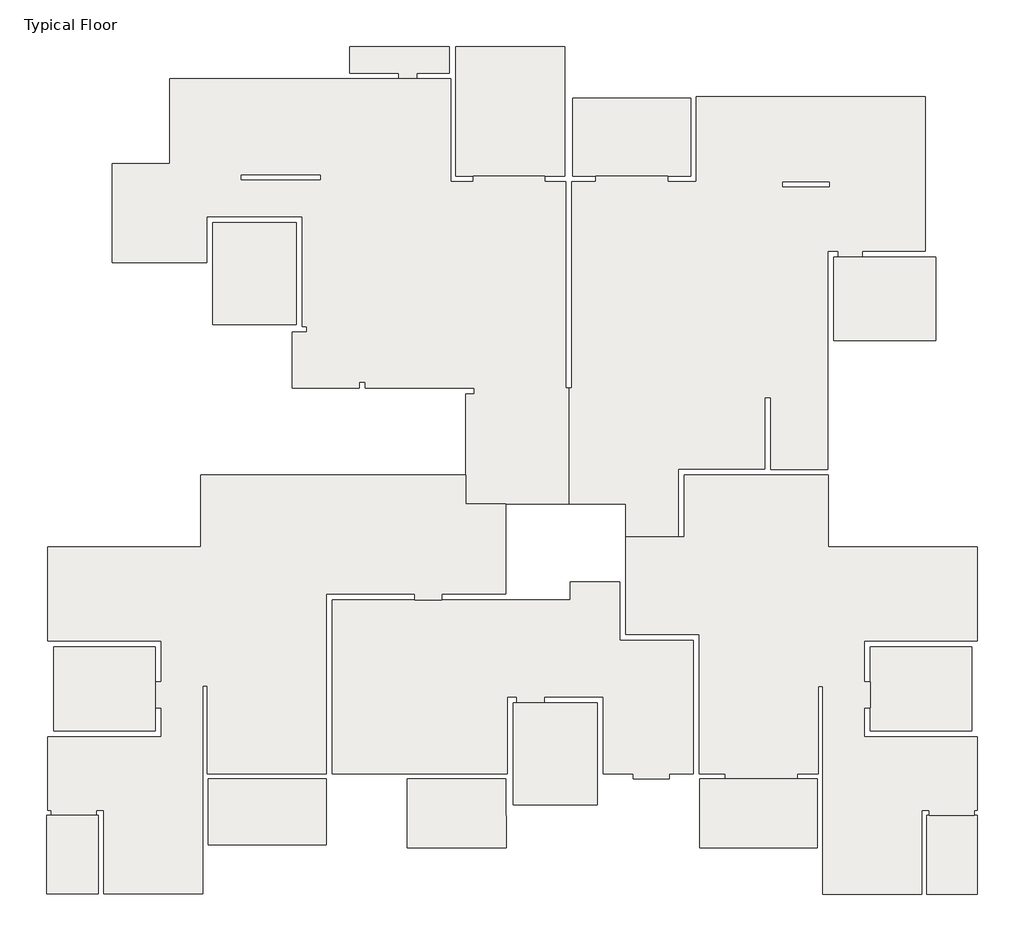
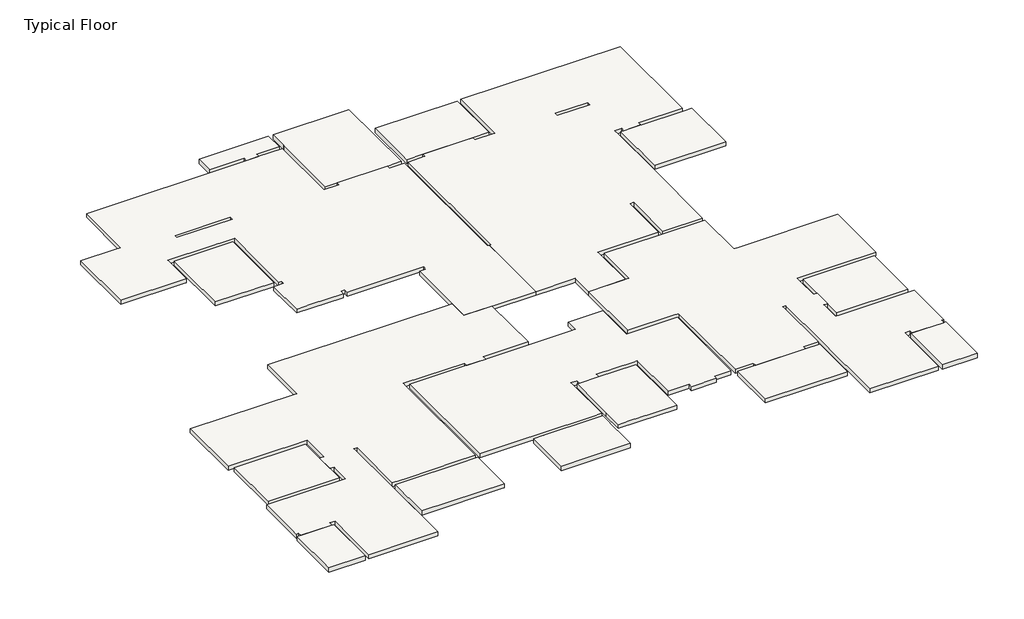
# One storey: 18 slabs.
"""IFC4 building model written with IfcOpenShell, lengths in millimetres."""

from ifc_helpers import new_model, si_unit, frame, origin, place, context, project, spatial, polyline, outline, extrude, faceted_brep, element, save

model = new_model("IFC4")

# Units and contexts
model_context = context("Model", 3, world=origin())
ifc_project = project(units=[si_unit("LENGTHUNIT", "METRE", prefix="MILLI")], contexts=[model_context])

# Site, building, storey
site = spatial("IfcSite", under=ifc_project)
building = spatial("IfcBuilding", under=site)
storey = spatial("IfcBuildingStorey", under=building, Name="Typical Floor", Elevation=3200.0)

# Slabs
placement = place(None, origin())
element("IfcSlab", 1, ObjectType="20", at=placement, inside=storey, context=model_context, shape_type="Brep", body=[
    faceted_brep([(-14926.2250005, -7113.2795537, 3000.0), (-14926.2250005, -8279.1882674, 3000.0), (-14926.2250005, -9149.744284, 3000.0), (-14926.2250005, -9913.0471886, 3000.0), (-18327.4781126, -9913.0471886, 3000.0), (-18327.4781126, -7113.2795537, 3000.0), (-14926.2250005, -7113.2795537, 3200.0), (-18327.4781126, -7113.2795537, 3200.0), (-18327.4781126, -9913.0471886, 3200.0), (-14926.2250005, -9913.0471886, 3200.0), (-14926.2250005, -9149.744284, 3200.0), (-14926.2250005, -8279.1882674, 3200.0)], [[[0, 1, 2, 3, 4, 5]], [[6, 7, 8, 9, 10, 11]], [[3, 2, 1, 0, 6, 11, 10, 9]], [[4, 3, 9, 8]], [[5, 4, 8, 7]], [[0, 5, 7, 6]]]),
])
element("IfcSlab", 2, ObjectType="20", at=placement, inside=storey, context=model_context, shape_type="Brep", body=[
    faceted_brep([(8945.0613065, -9913.0471886, 3000.0), (8945.0613065, -9149.744284, 3000.0), (8945.0613065, -8273.2795537, 3000.0), (8950.0364103, -8273.2795537, 3000.0), (8950.0364103, -7113.2795537, 3000.0), (12344.2065347, -7113.2795537, 3000.0), (12344.2065347, -9913.0471886, 3000.0), (8945.0613065, -8273.2795537, 3200.0), (8945.0613065, -9149.744284, 3200.0), (8945.0613065, -9913.0471886, 3200.0), (12344.2065347, -9913.0471886, 3200.0), (12344.2065347, -7113.2795537, 3200.0), (8950.0364103, -7113.2795537, 3200.0), (8950.0364103, -8273.2795537, 3200.0)], [[[0, 1, 2, 3, 4, 5, 6]], [[7, 8, 9, 10, 11, 12, 13]], [[9, 0, 6, 10]], [[0, 9, 8, 7, 2, 1]], [[4, 12, 11, 5]], [[3, 13, 12, 4]], [[13, 3, 2, 7]], [[6, 5, 11, 10]]]),
])
element("IfcSlab", 3, ObjectType="20", at=placement, inside=storey, context=model_context, shape_type="Brep", body=[
    faceted_brep([(-2966.5901458, -11344.051338, 3000.0), (-2966.5901458, -8982.9724998, 3000.0), (-2850.4075731, -8982.9724998, 3000.0), (-1944.0175316, -8982.9724998, 3000.0), (-164.9635897, -8982.9724998, 3000.0), (-164.9635897, -12384.2256118, 3000.0), (-2966.3411831, -12384.2256118, 3000.0), (-2966.3411831, -11344.051338, 3000.0), (-2966.5901458, -8982.9724998, 3200.0), (-2966.5901458, -11344.051338, 3200.0), (-2966.3411831, -11344.051338, 3200.0), (-2966.3411831, -11524.051338, 3200.0), (-2966.3411831, -12384.2256118, 3200.0), (-2445.6938802, -12384.2256118, 3200.0), (-1385.42832, -12384.2256118, 3200.0), (-164.9635897, -12384.2256118, 3200.0), (-164.9635897, -11524.051338, 3200.0), (-164.9635897, -11344.051338, 3200.0), (-164.9635897, -8982.9724998, 3200.0), (-1944.0175316, -8982.9724998, 3200.0), (-2850.4075731, -8982.9724998, 3200.0)], [[[0, 1, 2, 3, 4, 5, 6, 7]], [[8, 9, 10, 11, 12, 13, 14, 15, 16, 17, 18, 19, 20]], [[12, 6, 5, 15, 14, 13]], [[8, 1, 0, 9]], [[1, 8, 20, 19, 18, 4, 3, 2]], [[7, 10, 9, 0]], [[10, 7, 6, 12, 11]], [[15, 5, 4, 18, 17, 16]]]),
])
element("IfcSlab", 4, ObjectType="20", at=placement, inside=storey, context=model_context, shape_type="Brep", body=[
    faceted_brep([(11134.2812235, 3125.7328944, 3000.0), (7735.1359953, 3125.7328944, 3000.0), (7735.1359953, 5925.8407782, 3000.0), (7878.7210576, 5925.8407782, 3000.0), (7878.7210576, 5930.8407782, 3000.0), (8690.2563273, 5930.8407782, 3000.0), (8690.2563273, 5925.8407782, 3000.0), (11134.2812235, 5925.8407782, 3000.0), (7735.1359953, 3125.7328944, 3200.0), (11134.2812235, 3125.7328944, 3200.0), (11134.2812235, 5925.8407782, 3200.0), (10784.6629663, 5925.8407782, 3200.0), (8690.2563273, 5925.8407782, 3200.0), (8690.2563273, 5930.8407782, 3200.0), (7878.7210576, 5930.8407782, 3200.0), (7878.7210576, 5925.8407782, 3200.0), (7735.1359953, 5925.8407782, 3200.0)], [[[0, 1, 2, 3, 4, 5, 6, 7]], [[8, 9, 10, 11, 12, 13, 14, 15, 16]], [[13, 5, 4, 14]], [[9, 0, 7, 10]], [[1, 0, 9, 8]], [[1, 8, 16, 2]], [[10, 7, 6, 12, 11]], [[12, 6, 5, 13]], [[15, 3, 2, 16]], [[3, 15, 14, 4]]]),
])
element("IfcSlab", 5, ObjectType="20", at=placement, inside=storey, context=model_context, shape_type="Brep", body=[
    faceted_brep([(-10217.2125524, 7066.4548861, 3000.0), (-10217.2125524, 3666.4548861, 3000.0), (-13016.7312246, 3666.4548861, 3000.0), (-13016.7312246, 7066.4548861, 3000.0), (-10217.2125524, 3666.4548861, 3200.0), (-10217.2125524, 7066.4548861, 3200.0), (-13016.7312246, 7066.4548861, 3200.0), (-13016.7312246, 5736.9611102, 3200.0), (-13016.7312246, 3666.4548861, 3200.0)], [[[0, 1, 2, 3]], [[4, 5, 6, 7, 8]], [[1, 0, 5, 4]], [[1, 4, 8, 2]], [[5, 0, 3, 6]], [[2, 8, 7, 6, 3]]]),
])
element("IfcSlab", 6, ObjectType="20", at=placement, inside=storey, context=model_context, shape_type="Brep", body=[
    faceted_brep([(-9872.2125524, 3416.4548861, 3000.0), (-9872.2125524, 3596.4548861, 3000.0), (-10017.2125524, 3596.4548861, 3000.0), (-10017.2125524, 7066.4548861, 3000.0), (-10017.2125524, 7266.4548861, 3000.0), (-13016.7312246, 7266.4548861, 3000.0), (-13216.7312246, 7266.4548861, 3000.0), (-13216.7312246, 5736.9611102, 3000.0), (-13386.7312246, 5736.9611102, 3000.0), (-16367.4366188, 5736.9611102, 3000.0), (-16367.4366188, 9037.0772927, 3000.0), (-14627.1544611, 9037.0772927, 3000.0), (-14447.1544611, 9037.0772927, 3000.0), (-14447.1544611, 11886.1063384, 3000.0), (-5065.7934653, 11886.1063384, 3000.0), (-5065.7934653, 8617.6084131, 3000.0), (-5065.7934653, 8437.6084131, 3000.0), (-4315.3868263, 8437.6084131, 3000.0), (-4315.3868263, 8617.6084131, 3000.0), (-1916.615042, 8617.6084131, 3000.0), (-1916.615042, 8437.6084131, 3000.0), (-1246.7976146, 8437.6084131, 3000.0), (-1216.7976146, 8437.6084131, 3000.0), (-1216.7976146, 8435.2155047, 3000.0), (-1216.7976146, 1537.2266703, 3000.0), (-1116.7976146, 1537.2266703, 3000.0), (-1116.7976146, -2332.8480185, 3000.0), (-3216.9303947, -2332.8480185, 3000.0), (-4566.2250005, -2332.8480185, 3000.0), (-4566.2250005, -1364.051338, 3000.0), (-4566.2250005, -1089.1965662, 3000.0), (-4566.2250005, -39.4704251, 3000.0), (-4566.2250005, 1337.2266703, 3000.0), (-4266.9054985, 1337.2266703, 3000.0), (-4266.9054985, 1537.2266703, 3000.0), (-7916.2250005, 1537.2266703, 3000.0), (-7916.2250005, 1752.2266703, 3000.0), (-8116.2250005, 1752.2266703, 3000.0), (-8116.2250005, 1536.9777077, 3000.0), (-9666.1254155, 1536.9777077, 3000.0), (-10356.1254155, 1536.9777077, 3000.0), (-10356.1254155, 3416.4548861, 3000.0), (-10217.2125524, 3416.4548861, 3000.0), (-9416.4656644, 8666.4299898, 3000.0), (-12061.8598553, 8666.4299898, 3000.0), (-12061.8598553, 8516.4299898, 3000.0), (-9416.4656644, 8516.4299898, 3000.0), (-9872.2125524, 3596.4548861, 3200.0), (-9872.2125524, 3416.4548861, 3200.0), (-10217.2125524, 3416.4548861, 3200.0), (-10356.1254155, 3416.4548861, 3200.0), (-10356.1254155, 1536.9777077, 3200.0), (-9666.1254155, 1536.9777077, 3200.0), (-8116.2250005, 1536.9777077, 3200.0), (-8116.2250005, 1752.2266703, 3200.0), (-7916.2250005, 1752.2266703, 3200.0), (-7916.2250005, 1537.2266703, 3200.0), (-4266.9054985, 1537.2266703, 3200.0), (-4266.9054985, 1337.2266703, 3200.0), (-4566.2250005, 1337.2266703, 3200.0), (-4566.2250005, -39.4704251, 3200.0), (-4566.2250005, -1089.1965662, 3200.0), (-4566.2250005, -1364.051338, 3200.0), (-4566.2250005, -2332.8480185, 3200.0), (-3216.9303947, -2332.8480185, 3200.0), (-1116.7976146, -2332.8480185, 3200.0), (-1116.7976146, 1537.2266703, 3200.0), (-1216.7976146, 1537.2266703, 3200.0), (-1216.7976146, 8437.6084131, 3200.0), (-1916.615042, 8437.6084131, 3200.0), (-1916.615042, 8617.6084131, 3200.0), (-4315.3868263, 8617.6084131, 3200.0), (-4315.3868263, 8437.6084131, 3200.0), (-5065.7934653, 8437.6084131, 3200.0), (-5065.7934653, 8617.6084131, 3200.0), (-5065.7934653, 11886.1063384, 3200.0), (-6191.4034238, 11886.1063384, 3200.0), (-6790.0424279, 11886.1063384, 3200.0), (-14447.1544611, 11886.1063384, 3200.0), (-14447.1544611, 9037.0772927, 3200.0), (-14627.1544611, 9037.0772927, 3200.0), (-16367.4366188, 9037.0772927, 3200.0), (-16367.4366188, 5736.9611102, 3200.0), (-13386.7312246, 5736.9611102, 3200.0), (-13216.7312246, 5736.9611102, 3200.0), (-13216.7312246, 7266.4548861, 3200.0), (-13016.7312246, 7266.4548861, 3200.0), (-10017.2125524, 7266.4548861, 3200.0), (-10017.2125524, 7066.4548861, 3200.0), (-10017.2125524, 3596.4548861, 3200.0), (-12061.8598553, 8666.4299898, 3200.0), (-9416.4656644, 8666.4299898, 3200.0), (-9416.4656644, 8516.4299898, 3200.0), (-12061.8598553, 8516.4299898, 3200.0)], [[[0, 1, 2, 3, 4, 5, 6, 7, 8, 9, 10, 11, 12, 13, 14, 15, 16, 17, 18, 19, 20, 21, 22, 23, 24, 25, 26, 27, 28, 29, 30, 31, 32, 33, 34, 35, 36, 37, 38, 39, 40, 41, 42], [43, 44, 45, 46]], [[47, 48, 49, 50, 51, 52, 53, 54, 55, 56, 57, 58, 59, 60, 61, 62, 63, 64, 65, 66, 67, 68, 69, 70, 71, 72, 73, 74, 75, 76, 77, 78, 79, 80, 81, 82, 83, 84, 85, 86, 87, 88, 89], [90, 91, 92, 93]], [[48, 0, 42, 41, 50, 49]], [[1, 0, 48, 47]], [[2, 1, 47, 89]], [[2, 89, 88, 87, 4, 3]], [[4, 87, 86, 85, 6, 5]], [[7, 6, 85, 84]], [[7, 84, 83, 82, 9, 8]], [[10, 9, 82, 81]], [[10, 81, 80, 79, 12, 11]], [[13, 12, 79, 78]], [[14, 13, 78, 77, 76, 75]], [[14, 75, 74, 73, 16, 15]], [[17, 16, 73, 72]], [[18, 17, 72, 71]], [[19, 18, 71, 70]], [[20, 19, 70, 69]], [[22, 21, 20, 69, 68]], [[24, 23, 22, 68, 67]], [[25, 24, 67, 66]], [[26, 25, 66, 65]], [[28, 27, 26, 65, 64, 63]], [[28, 63, 62, 61, 60, 59, 32, 31, 30, 29]], [[33, 32, 59, 58]], [[34, 33, 58, 57]], [[35, 34, 57, 56]], [[36, 35, 56, 55]], [[37, 36, 55, 54]], [[38, 37, 54, 53]], [[38, 53, 52, 51, 40, 39]], [[41, 40, 51, 50]], [[44, 43, 91, 90]], [[45, 44, 90, 93]], [[46, 45, 93, 92]], [[43, 46, 92, 91]]]),
])
element("IfcSlab", 7, ObjectType="20", at=placement, inside=storey, context=model_context, shape_type="Brep", body=[
    faceted_brep([(-13417.2291499, -1364.051338, 3000.0), (-4566.2250005, -1364.051338, 3000.0), (-4566.2250005, -2332.8480185, 3000.0), (-3216.9303947, -2332.8480185, 3000.0), (-3216.9303947, -5334.7235371, 3000.0), (-5367.2208511, -5334.7235371, 3000.0), (-5367.2208511, -5534.7235371, 3000.0), (-6267.2872412, -5534.7235371, 3000.0), (-6267.2872412, -5334.7235371, 3000.0), (-9216.2167018, -5334.7235371, 3000.0), (-9216.2167018, -5534.7235371, 3000.0), (-9216.2167018, -11344.051338, 3000.0), (-10116.2830918, -11344.051338, 3000.0), (-12517.1627599, -11344.051338, 3000.0), (-13197.6689839, -11344.051338, 3000.0), (-13197.6689839, -8414.0928317, 3000.0), (-13347.6689839, -8414.0928317, 3000.0), (-13347.6689839, -11344.051338, 3000.0), (-13347.6689839, -11524.051338, 3000.0), (-13347.6689839, -15365.0637861, 3000.0), (-16646.5071582, -15365.0637861, 3000.0), (-16646.5071582, -12744.5160683, 3000.0), (-16646.5071582, -12564.5160683, 3000.0), (-16907.8847516, -12564.5160683, 3000.0), (-16907.8847516, -12744.5160683, 3000.0), (-18406.5901458, -12744.5160683, 3000.0), (-18406.5901458, -12564.5160683, 3000.0), (-18517.4781126, -12564.5160683, 3000.0), (-18517.4781126, -10113.0471886, 3000.0), (-14726.2250005, -10113.0471886, 3000.0), (-14726.2250005, -9913.0471886, 3000.0), (-14726.2250005, -9149.744284, 3000.0), (-14926.2250005, -9149.744284, 3000.0), (-14926.2250005, -8279.1882674, 3000.0), (-14726.2250005, -8279.1882674, 3000.0), (-14726.2250005, -6913.2795537, 3000.0), (-14926.2250005, -6913.2795537, 3000.0), (-18517.4781126, -6913.2795537, 3000.0), (-18517.4781126, -3764.1011305, 3000.0), (-13417.2291499, -3764.1011305, 3000.0), (-13417.2291499, -3584.1011305, 3000.0), (-4566.2250005, -1364.051338, 3200.0), (-4766.2250005, -1364.051338, 3200.0), (-9767.2291499, -1364.051338, 3200.0), (-13417.2291499, -1364.051338, 3200.0), (-13417.2291499, -3584.1011305, 3200.0), (-13417.2291499, -3764.1011305, 3200.0), (-18517.4781126, -3764.1011305, 3200.0), (-18517.4781126, -6913.2795537, 3200.0), (-14926.2250005, -6913.2795537, 3200.0), (-14726.2250005, -6913.2795537, 3200.0), (-14726.2250005, -8279.1882674, 3200.0), (-14926.2250005, -8279.1882674, 3200.0), (-14926.2250005, -9149.744284, 3200.0), (-14726.2250005, -9149.744284, 3200.0), (-14726.2250005, -9913.0471886, 3200.0), (-14726.2250005, -10113.0471886, 3200.0), (-18517.4781126, -10113.0471886, 3200.0), (-18517.4781126, -12564.5160683, 3200.0), (-18406.5901458, -12564.5160683, 3200.0), (-18406.5901458, -12744.5160683, 3200.0), (-16907.8847516, -12744.5160683, 3200.0), (-16907.8847516, -12564.5160683, 3200.0), (-16646.5071582, -12564.5160683, 3200.0), (-16646.5071582, -12744.5160683, 3200.0), (-16646.5071582, -15365.0637861, 3200.0), (-13347.6689839, -15365.0637861, 3200.0), (-13347.6689839, -11524.051338, 3200.0), (-13347.6689839, -11344.051338, 3200.0), (-13347.6689839, -8414.0928317, 3200.0), (-13197.6689839, -8414.0928317, 3200.0), (-13197.6689839, -11344.051338, 3200.0), (-12517.1627599, -11344.051338, 3200.0), (-10116.2830918, -11344.051338, 3200.0), (-9216.2167018, -11344.051338, 3200.0), (-9216.2167018, -5534.7235371, 3200.0), (-9216.2167018, -5334.7235371, 3200.0), (-6267.2872412, -5334.7235371, 3200.0), (-6267.2872412, -5534.7235371, 3200.0), (-5367.2208511, -5534.7235371, 3200.0), (-5367.2208511, -5334.7235371, 3200.0), (-3216.9303947, -5334.7235371, 3200.0), (-3216.9303947, -2332.8480185, 3200.0), (-4566.2250005, -2332.8480185, 3200.0)], [[[0, 1, 2, 3, 4, 5, 6, 7, 8, 9, 10, 11, 12, 13, 14, 15, 16, 17, 18, 19, 20, 21, 22, 23, 24, 25, 26, 27, 28, 29, 30, 31, 32, 33, 34, 35, 36, 37, 38, 39, 40]], [[41, 42, 43, 44, 45, 46, 47, 48, 49, 50, 51, 52, 53, 54, 55, 56, 57, 58, 59, 60, 61, 62, 63, 64, 65, 66, 67, 68, 69, 70, 71, 72, 73, 74, 75, 76, 77, 78, 79, 80, 81, 82, 83]], [[1, 0, 44, 43, 42, 41]], [[2, 1, 41, 83]], [[3, 2, 83, 82]], [[4, 3, 82, 81]], [[5, 4, 81, 80]], [[6, 5, 80, 79]], [[7, 6, 79, 78]], [[8, 7, 78, 77]], [[9, 8, 77, 76]], [[9, 76, 75, 74, 11, 10]], [[11, 74, 73, 72, 71, 14, 13, 12]], [[15, 14, 71, 70]], [[16, 15, 70, 69]], [[16, 69, 68, 67, 66, 19, 18, 17]], [[20, 19, 66, 65]], [[20, 65, 64, 63, 22, 21]], [[23, 22, 63, 62]], [[24, 23, 62, 61]], [[25, 24, 61, 60]], [[26, 25, 60, 59]], [[27, 26, 59, 58]], [[28, 27, 58, 57]], [[29, 28, 57, 56]], [[29, 56, 55, 54, 31, 30]], [[32, 31, 54, 53]], [[33, 32, 53, 52]], [[34, 33, 52, 51]], [[35, 34, 51, 50]], [[35, 50, 49, 48, 37, 36]], [[38, 37, 48, 47]], [[39, 38, 47, 46]], [[39, 46, 45, 44, 0, 40]]]),
])
element("IfcSlab", 8, ObjectType="20", at=placement, inside=storey, context=model_context, shape_type="Brep", body=[
    faceted_brep([(-1116.7976146, 1537.2266703, 3000.0), (-1016.7976146, 1537.2266703, 3000.0), (-1016.7976146, 8437.6084131, 3000.0), (-215.5528014, 8437.6084131, 3000.0), (-215.5528014, 8617.6084131, 3000.0), (2183.2189829, 8617.6084131, 3000.0), (2183.2189829, 8437.6084131, 3000.0), (3133.8745845, 8437.6084131, 3000.0), (3133.8745845, 8617.6084131, 3000.0), (3133.8745845, 11276.9279151, 3000.0), (10784.6629663, 11276.9279151, 3000.0), (10784.6629663, 6125.8407782, 3000.0), (8690.2563273, 6125.8407782, 3000.0), (8690.2563273, 5930.8407782, 3000.0), (7878.7210576, 5930.8407782, 3000.0), (7878.7210576, 6125.8407782, 3000.0), (7535.1359953, 6125.8407782, 3000.0), (7535.1359953, 5925.8407782, 3000.0), (7535.1359953, 2875.7328944, 3000.0), (7535.1359953, -1184.051338, 3000.0), (5633.824792, -1184.051338, 3000.0), (5633.824792, 1223.1519815, 3000.0), (5433.824792, 1223.1519815, 3000.0), (5433.824792, -1164.051338, 3000.0), (2535.2355804, -1164.051338, 3000.0), (2535.2355804, -1364.051338, 3000.0), (2535.2355804, -3433.1633712, 3000.0), (783.3351654, -3433.1633712, 3000.0), (783.3351654, -2332.8480185, 3000.0), (583.3351654, -2332.8480185, 3000.0), (-1116.7976146, -2332.8480185, 3000.0), (7585.7252069, 8425.7909857, 3000.0), (6036.4306011, 8425.7909857, 3000.0), (6036.4306011, 8275.7909857, 3000.0), (7585.7252069, 8275.7909857, 3000.0), (-1016.7976146, 1537.2266703, 3200.0), (-1116.7976146, 1537.2266703, 3200.0), (-1116.7976146, -2332.8480185, 3200.0), (583.3351654, -2332.8480185, 3200.0), (783.3351654, -2332.8480185, 3200.0), (783.3351654, -3433.1633712, 3200.0), (2535.2355804, -3433.1633712, 3200.0), (2535.2355804, -1364.051338, 3200.0), (2535.2355804, -1164.051338, 3200.0), (5433.824792, -1164.051338, 3200.0), (5433.824792, 1223.1519815, 3200.0), (5633.824792, 1223.1519815, 3200.0), (5633.824792, -1184.051338, 3200.0), (7535.1359953, -1184.051338, 3200.0), (7535.1359953, 2875.7328944, 3200.0), (7535.1359953, 5925.8407782, 3200.0), (7535.1359953, 6125.8407782, 3200.0), (7878.7210576, 6125.8407782, 3200.0), (7878.7210576, 5930.8407782, 3200.0), (8690.2563273, 5930.8407782, 3200.0), (8690.2563273, 6125.8407782, 3200.0), (10784.6629663, 6125.8407782, 3200.0), (10784.6629663, 6175.8407782, 3200.0), (10784.6629663, 11276.9279151, 3200.0), (3133.8745845, 11276.9279151, 3200.0), (3133.8745845, 8617.6084131, 3200.0), (3133.8745845, 8437.6084131, 3200.0), (2183.2189829, 8437.6084131, 3200.0), (2183.2189829, 8617.6084131, 3200.0), (-215.5528014, 8617.6084131, 3200.0), (-215.5528014, 8437.6084131, 3200.0), (-1016.7976146, 8437.6084131, 3200.0), (6036.4306011, 8425.7909857, 3200.0), (7585.7252069, 8425.7909857, 3200.0), (7585.7252069, 8275.7909857, 3200.0), (6036.4306011, 8275.7909857, 3200.0)], [[[0, 1, 2, 3, 4, 5, 6, 7, 8, 9, 10, 11, 12, 13, 14, 15, 16, 17, 18, 19, 20, 21, 22, 23, 24, 25, 26, 27, 28, 29, 30], [31, 32, 33, 34]], [[35, 36, 37, 38, 39, 40, 41, 42, 43, 44, 45, 46, 47, 48, 49, 50, 51, 52, 53, 54, 55, 56, 57, 58, 59, 60, 61, 62, 63, 64, 65, 66], [67, 68, 69, 70]], [[1, 0, 36, 35]], [[2, 1, 35, 66]], [[3, 2, 66, 65]], [[4, 3, 65, 64]], [[5, 4, 64, 63]], [[6, 5, 63, 62]], [[7, 6, 62, 61]], [[7, 61, 60, 59, 9, 8]], [[10, 9, 59, 58]], [[11, 10, 58, 57, 56]], [[12, 11, 56, 55]], [[12, 55, 54, 13]], [[52, 15, 14, 53]], [[16, 15, 52, 51]], [[16, 51, 50, 49, 18, 17]], [[20, 19, 48, 47]], [[21, 20, 47, 46]], [[22, 21, 46, 45]], [[23, 22, 45, 44]], [[24, 23, 44, 43]], [[24, 43, 42, 41, 26, 25]], [[27, 26, 41, 40]], [[28, 27, 40, 39]], [[28, 39, 38, 37, 30, 29]], [[0, 30, 37, 36]], [[19, 18, 49, 48]], [[32, 31, 68, 67]], [[33, 32, 67, 70]], [[34, 33, 70, 69]], [[31, 34, 69, 68]], [[14, 13, 54, 53]]]),
])
element("IfcSlab", 9, ObjectType="20", at=placement, inside=storey, context=model_context, shape_type="Brep", body=[
    faceted_brep([(2735.2355804, -3433.1633712, 3000.0), (2735.2355804, -1364.051338, 3000.0), (7555.384958, -1364.051338, 3000.0), (7555.384958, -3764.1011305, 3000.0), (7735.384958, -3764.1011305, 3000.0), (12534.2065347, -3764.1011305, 3000.0), (12534.2065347, -6913.2795537, 3000.0), (8750.0364103, -6913.2795537, 3000.0), (8750.0364103, -7113.2795537, 3000.0), (8750.0364103, -8273.2795537, 3000.0), (8945.0613065, -8273.2795537, 3000.0), (8945.0613065, -9149.744284, 3000.0), (8745.0613065, -9149.744284, 3000.0), (8745.0613065, -10113.0471886, 3000.0), (8945.0613065, -10113.0471886, 3000.0), (12534.2065347, -10113.0471886, 3000.0), (12534.2065347, -12564.5160683, 3000.0), (12429.6422194, -12564.5160683, 3000.0), (12429.6422194, -12744.5160683, 3000.0), (10930.9368252, -12744.5160683, 3000.0), (10930.9368252, -12564.5160683, 3000.0), (10665.3434642, -12564.5160683, 3000.0), (10665.3434642, -12744.5160683, 3000.0), (10665.3434642, -15369.5160683, 3000.0), (7365.3434642, -15369.5160683, 3000.0), (7365.3434642, -11434.051338, 3000.0), (7365.3434642, -8419.051338, 3000.0), (7215.3434642, -8419.051338, 3000.0), (7215.3434642, -11344.051338, 3000.0), (6514.9202277, -11344.051338, 3000.0), (6514.9202277, -11524.051338, 3000.0), (4114.0405596, -11524.051338, 3000.0), (4114.0405596, -11344.051338, 3000.0), (3235.0530078, -11344.051338, 3000.0), (3235.0530078, -6683.5202176, 3000.0), (3035.0530078, -6683.5202176, 3000.0), (783.3351654, -6683.5202176, 3000.0), (783.3351654, -3433.1633712, 3000.0), (2535.2355804, -3433.1633712, 3000.0), (2735.2355804, -1364.051338, 3200.0), (2735.2355804, -3433.1633712, 3200.0), (2535.2355804, -3433.1633712, 3200.0), (783.3351654, -3433.1633712, 3200.0), (783.3351654, -6683.5202176, 3200.0), (3035.0530078, -6683.5202176, 3200.0), (3235.0530078, -6683.5202176, 3200.0), (3235.0530078, -11344.051338, 3200.0), (4114.0405596, -11344.051338, 3200.0), (4114.0405596, -11524.051338, 3200.0), (6514.9202277, -11524.051338, 3200.0), (6514.9202277, -11344.051338, 3200.0), (7215.3434642, -11344.051338, 3200.0), (7215.3434642, -8419.051338, 3200.0), (7365.3434642, -8419.051338, 3200.0), (7365.3434642, -11434.051338, 3200.0), (7365.3434642, -15369.5160683, 3200.0), (10665.3434642, -15369.5160683, 3200.0), (10665.3434642, -12744.5160683, 3200.0), (10665.3434642, -12564.5160683, 3200.0), (10930.9368252, -12564.5160683, 3200.0), (10930.9368252, -12744.5160683, 3200.0), (12429.6422194, -12744.5160683, 3200.0), (12429.6422194, -12564.5160683, 3200.0), (12534.2065347, -12564.5160683, 3200.0), (12534.2065347, -10113.0471886, 3200.0), (8945.0613065, -10113.0471886, 3200.0), (8745.0613065, -10113.0471886, 3200.0), (8745.0613065, -9149.744284, 3200.0), (8945.0613065, -9149.744284, 3200.0), (8945.0613065, -8273.2795537, 3200.0), (8750.0364103, -8273.2795537, 3200.0), (8750.0364103, -7113.2795537, 3200.0), (8750.0364103, -6913.2795537, 3200.0), (12534.2065347, -6913.2795537, 3200.0), (12534.2065347, -3764.1011305, 3200.0), (7735.384958, -3764.1011305, 3200.0), (7555.384958, -3764.1011305, 3200.0), (7555.384958, -1364.051338, 3200.0), (5433.824792, -1364.051338, 3200.0)], [[[0, 1, 2, 3, 4, 5, 6, 7, 8, 9, 10, 11, 12, 13, 14, 15, 16, 17, 18, 19, 20, 21, 22, 23, 24, 25, 26, 27, 28, 29, 30, 31, 32, 33, 34, 35, 36, 37, 38]], [[39, 40, 41, 42, 43, 44, 45, 46, 47, 48, 49, 50, 51, 52, 53, 54, 55, 56, 57, 58, 59, 60, 61, 62, 63, 64, 65, 66, 67, 68, 69, 70, 71, 72, 73, 74, 75, 76, 77, 78]], [[1, 0, 40, 39]], [[2, 1, 39, 78, 77]], [[3, 2, 77, 76]], [[3, 76, 75, 74, 5, 4]], [[6, 5, 74, 73]], [[7, 6, 73, 72]], [[7, 72, 71, 70, 9, 8]], [[9, 70, 69, 10]], [[67, 12, 11, 68]], [[13, 12, 67, 66]], [[13, 66, 65, 64, 15, 14]], [[16, 15, 64, 63]], [[17, 16, 63, 62]], [[18, 17, 62, 61]], [[19, 18, 61, 60]], [[20, 19, 60, 59]], [[21, 20, 59, 58]], [[21, 58, 57, 56, 23, 22]], [[24, 23, 56, 55]], [[24, 55, 54, 53, 26, 25]], [[27, 26, 53, 52]], [[28, 27, 52, 51]], [[29, 28, 51, 50]], [[30, 29, 50, 49]], [[31, 30, 49, 48]], [[32, 31, 48, 47]], [[33, 32, 47, 46]], [[34, 33, 46, 45]], [[34, 45, 44, 43, 36, 35]], [[37, 36, 43, 42]], [[37, 42, 41, 40, 0, 38]], [[11, 10, 69, 68]]]),
])
element("IfcSlab", 10, ObjectType="20", at=placement, inside=storey, context=model_context, shape_type="Brep", body=[
    faceted_brep([(-9016.2167018, -11344.051338, 3000.0), (-9016.2167018, -5534.7235371, 3000.0), (-6267.2872412, -5534.7235371, 3000.0), (-5367.2208511, -5534.7235371, 3000.0), (-1265.2789424, -5534.7235371, 3000.0), (-1065.2789424, -5534.7235371, 3000.0), (-1065.2789424, -4933.7276865, 3000.0), (583.3351654, -4933.7276865, 3000.0), (583.3351654, -6683.5202176, 3000.0), (583.3351654, -6883.5202176, 3000.0), (3035.0530078, -6883.5202176, 3000.0), (3035.0530078, -11344.051338, 3000.0), (2233.8081945, -11344.051338, 3000.0), (2233.8081945, -11524.051338, 3000.0), (1034.4223024, -11524.051338, 3000.0), (1034.4223024, -11344.051338, 3000.0), (35.0364103, -11344.051338, 3000.0), (35.0364103, -8782.9724998, 3000.0), (-164.9635897, -8782.9724998, 3000.0), (-1944.0175316, -8782.9724998, 3000.0), (-1944.0175316, -8982.9724998, 3000.0), (-2850.4075731, -8982.9724998, 3000.0), (-2850.4075731, -8782.9724998, 3000.0), (-3166.5901458, -8782.9724998, 3000.0), (-3166.5901458, -8982.9724998, 3000.0), (-3166.5901458, -11344.051338, 3000.0), (-3636.648237, -11344.051338, 3000.0), (-6035.4200213, -11344.051338, 3000.0), (-7066.175208, -11344.051338, 3000.0), (-8566.988486, -11344.051338, 3000.0), (-9016.2167018, -5534.7235371, 3200.0), (-9016.2167018, -11344.051338, 3200.0), (-8566.988486, -11344.051338, 3200.0), (-7066.175208, -11344.051338, 3200.0), (-6035.4200213, -11344.051338, 3200.0), (-3636.648237, -11344.051338, 3200.0), (-3166.5901458, -11344.051338, 3200.0), (-3166.5901458, -8982.9724998, 3200.0), (-3166.5901458, -8782.9724998, 3200.0), (-2850.4075731, -8782.9724998, 3200.0), (-2850.4075731, -8982.9724998, 3200.0), (-1944.0175316, -8982.9724998, 3200.0), (-1944.0175316, -8782.9724998, 3200.0), (-164.9635897, -8782.9724998, 3200.0), (35.0364103, -8782.9724998, 3200.0), (35.0364103, -11344.051338, 3200.0), (1034.4223024, -11344.051338, 3200.0), (1034.4223024, -11524.051338, 3200.0), (2233.8081945, -11524.051338, 3200.0), (2233.8081945, -11344.051338, 3200.0), (3035.0530078, -11344.051338, 3200.0), (3035.0530078, -6883.5202176, 3200.0), (583.3351654, -6883.5202176, 3200.0), (583.3351654, -6683.5202176, 3200.0), (583.3351654, -4933.7276865, 3200.0), (-1065.2789424, -4933.7276865, 3200.0), (-1065.2789424, -5534.7235371, 3200.0), (-1265.2789424, -5534.7235371, 3200.0), (-5367.2208511, -5534.7235371, 3200.0), (-6267.2872412, -5534.7235371, 3200.0)], [[[0, 1, 2, 3, 4, 5, 6, 7, 8, 9, 10, 11, 12, 13, 14, 15, 16, 17, 18, 19, 20, 21, 22, 23, 24, 25, 26, 27, 28, 29]], [[30, 31, 32, 33, 34, 35, 36, 37, 38, 39, 40, 41, 42, 43, 44, 45, 46, 47, 48, 49, 50, 51, 52, 53, 54, 55, 56, 57, 58, 59]], [[1, 0, 31, 30]], [[1, 30, 59, 58, 3, 2]], [[3, 58, 57, 56, 5, 4]], [[6, 5, 56, 55]], [[7, 6, 55, 54]], [[7, 54, 53, 52, 9, 8]], [[10, 9, 52, 51]], [[11, 10, 51, 50]], [[12, 11, 50, 49]], [[13, 12, 49, 48]], [[14, 13, 48, 47]], [[15, 14, 47, 46]], [[16, 15, 46, 45]], [[17, 16, 45, 44]], [[17, 44, 43, 42, 19, 18]], [[20, 19, 42, 41]], [[21, 20, 41, 40]], [[22, 21, 40, 39]], [[23, 22, 39, 38]], [[23, 38, 37, 36, 25, 24]], [[25, 36, 35, 34, 33, 32, 31, 0, 29, 28, 27, 26]]]),
])
element("IfcSlab", 11, ObjectType="22", at=placement, inside=storey, context=model_context, shape_type="Brep", body=[
    faceted_brep([(-16826.5071582, -15365.0637861, 2980.0), (-18561.2442958, -15365.0637861, 2980.0), (-18561.2442958, -12744.5160683, 2980.0), (-16826.5071582, -12744.5160683, 2980.0), (-16826.5071582, -15365.0637861, 3200.0), (-16826.5071582, -12744.5160683, 3200.0), (-16907.8847516, -12744.5160683, 3200.0), (-18406.5901458, -12744.5160683, 3200.0), (-18561.2442958, -12744.5160683, 3200.0), (-18561.2442958, -15365.0637861, 3200.0)], [[[0, 1, 2, 3]], [[4, 5, 6, 7, 8, 9]], [[1, 0, 4, 9]], [[2, 1, 9, 8]], [[3, 2, 8, 7, 6, 5]], [[0, 3, 5, 4]]]),
])
element("IfcSlab", 12, ObjectType="22", at=placement, inside=storey, context=model_context, shape_type="Brep", body=[
    faceted_brep([(12534.2065347, -12744.5160683, 2980.0), (12534.2065347, -15369.5160683, 2980.0), (10845.3434642, -15369.5160683, 2980.0), (10845.3434642, -12744.5160683, 2980.0), (12534.2065347, -12744.5160683, 3200.0), (12429.6422194, -12744.5160683, 3200.0), (10930.9368252, -12744.5160683, 3200.0), (10845.3434642, -12744.5160683, 3200.0), (10845.3434642, -15369.5160683, 3200.0), (12534.2065347, -15369.5160683, 3200.0)], [[[0, 1, 2, 3]], [[4, 5, 6, 7, 8, 9]], [[1, 0, 4, 9]], [[2, 1, 9, 8]], [[3, 2, 8, 7]], [[0, 3, 7, 6, 5, 4]]]),
])
element("IfcSlab", 13, ObjectType="22", at=placement, inside=storey, context=model_context, shape_type="Brep", body=[
    faceted_brep([(-3211.3411831, -13814.491172, 2980.0), (-3220.4458666, -13814.491172, 2980.0), (-6516.0175316, -13814.491172, 2980.0), (-6516.0175316, -11524.051338, 2980.0), (-6035.4200213, -11524.051338, 2980.0), (-6035.4200213, -11519.051338, 2980.0), (-3636.648237, -11519.051338, 2980.0), (-3636.648237, -11524.051338, 2980.0), (-3216.3411831, -11524.051338, 2980.0), (-3216.3411831, -12636.8603469, 2980.0), (-3216.3411831, -12754.2256118, 2980.0), (-3211.3411831, -12754.2256118, 2980.0), (-6516.0175316, -13814.491172, 3200.0), (-3220.4458666, -13814.491172, 3200.0), (-3211.3411831, -13814.491172, 3200.0), (-3211.3411831, -12754.2256118, 3200.0), (-3216.3411831, -12754.2256118, 3200.0), (-3216.3411831, -11524.051338, 3200.0), (-3636.648237, -11524.051338, 3200.0), (-3636.648237, -11519.051338, 3200.0), (-6035.4200213, -11519.051338, 3200.0), (-6035.4200213, -11524.051338, 3200.0), (-6516.0175316, -11524.051338, 3200.0), (-6516.0175316, -13068.3003006, 3200.0)], [[[0, 1, 2, 3, 4, 5, 6, 7, 8, 9, 10, 11]], [[12, 13, 14, 15, 16, 17, 18, 19, 20, 21, 22, 23]], [[14, 0, 11, 15]], [[2, 1, 0, 14, 13, 12]], [[2, 12, 23, 22, 3]], [[19, 6, 5, 20]], [[7, 18, 17, 8]], [[18, 7, 6, 19]], [[21, 4, 3, 22]], [[4, 21, 20, 5]], [[16, 10, 9, 8, 17]], [[10, 16, 15, 11]]]),
])
element("IfcSlab", 14, ObjectType="22", at=placement, inside=storey, context=model_context, shape_type="Brep", body=[
    faceted_brep([(7185.3434642, -11524.051338, 2980.0), (7185.3434642, -13814.491172, 2980.0), (3265.0530078, -13814.491172, 2980.0), (3265.0530078, -11524.051338, 2980.0), (7185.3434642, -13814.491172, 3200.0), (7185.3434642, -11524.051338, 3200.0), (6514.9202277, -11524.051338, 3200.0), (4114.0405596, -11524.051338, 3200.0), (3265.0530078, -11524.051338, 3200.0), (3265.0530078, -13814.491172, 3200.0)], [[[0, 1, 2, 3]], [[4, 5, 6, 7, 8, 9]], [[1, 0, 5, 4]], [[2, 1, 4, 9]], [[3, 2, 9, 8]], [[0, 3, 8, 7, 6, 5]]]),
])
element("IfcSlab", 15, ObjectType="22", at=placement, inside=storey, context=model_context, shape_type="Brep", body=[
    faceted_brep([(-9211.2167018, -13713.3127488, 2980.0), (-9216.2167018, -13713.3127488, 2980.0), (-13167.6689839, -13713.3127488, 2980.0), (-13167.6689839, -11524.051338, 2980.0), (-9216.2167018, -11524.051338, 2980.0), (-9216.2167018, -13068.3003006, 2980.0), (-9211.2167018, -13068.3003006, 2980.0), (-13167.6689839, -13713.3127488, 3200.0), (-9211.2167018, -13713.3127488, 3200.0), (-9211.2167018, -13068.3003006, 3200.0), (-9216.2167018, -13068.3003006, 3200.0), (-9216.2167018, -11524.051338, 3200.0), (-10116.2830918, -11524.051338, 3200.0), (-12517.1627599, -11524.051338, 3200.0), (-13167.6689839, -11524.051338, 3200.0)], [[[0, 1, 2, 3, 4, 5, 6]], [[7, 8, 9, 10, 11, 12, 13, 14]], [[8, 0, 6, 9]], [[2, 1, 0, 8, 7]], [[3, 2, 7, 14]], [[3, 14, 13, 12, 11, 4]], [[10, 5, 4, 11]], [[5, 10, 9, 6]]]),
])
element("IfcSlab", 16, ObjectType="22", at=placement, inside=storey, context=model_context, shape_type="SweptSolid", body=[
    extrude(outline(polyline([(-8435.5693989, 12957.7411932), (-5116.3826769, 12957.7411932), (-5116.3826769, 12066.1063384), (-6191.4034238, 12066.1063384), (-6191.4034238, 11886.1063384), (-6790.0424279, 11886.1063384), (-6790.0424279, 12066.1063384), (-8435.5693989, 12066.1063384), (-8435.5693989, 12957.7411932)])), frame((0.0, 0.0, 2980.0), z_axis=(0.0, 0.0, 1.0), x_axis=(1.0, 0.0, 0.0)), (0.0, 0.0, 1.0), 220.0),
])
element("IfcSlab", 17, ObjectType="22", at=placement, inside=storey, context=model_context, shape_type="Brep", body=[
    faceted_brep([(-1246.7976146, 12957.7411932, 2980.0), (-1246.7976146, 8617.6084131, 2980.0), (-4885.7934653, 8617.6084131, 2980.0), (-4885.7934653, 12066.1063384, 2980.0), (-4886.3826769, 12066.1063384, 2980.0), (-4886.3826769, 12957.7411932, 2980.0), (-1246.7976146, 8617.6084131, 3200.0), (-1246.7976146, 12957.7411932, 3200.0), (-4886.3826769, 12957.7411932, 3200.0), (-4886.3826769, 12066.1063384, 3200.0), (-4885.7934653, 12066.1063384, 3200.0), (-4885.7934653, 8617.6084131, 3200.0), (-4315.3868263, 8617.6084131, 3200.0), (-1916.615042, 8617.6084131, 3200.0)], [[[0, 1, 2, 3, 4, 5]], [[6, 7, 8, 9, 10, 11, 12, 13]], [[1, 0, 7, 6]], [[1, 6, 13, 12, 11, 2]], [[8, 5, 4, 9]], [[0, 5, 8, 7]], [[10, 3, 2, 11]], [[3, 10, 9, 4]]]),
])
element("IfcSlab", 18, ObjectType="22", at=placement, inside=storey, context=model_context, shape_type="Brep", body=[
    faceted_brep([(2953.8745845, 11237.7079981, 2980.0), (2953.8745845, 8617.6084131, 2980.0), (-986.7976146, 8617.6084131, 2980.0), (-986.7976146, 11237.7079981, 2980.0), (2953.8745845, 8617.6084131, 3200.0), (2953.8745845, 11237.7079981, 3200.0), (-986.7976146, 11237.7079981, 3200.0), (-986.7976146, 8617.6084131, 3200.0), (-215.5528014, 8617.6084131, 3200.0), (2183.2189829, 8617.6084131, 3200.0)], [[[0, 1, 2, 3]], [[4, 5, 6, 7, 8, 9]], [[1, 0, 5, 4]], [[2, 1, 4, 9, 8, 7]], [[3, 2, 7, 6]], [[0, 3, 6, 5]]]),
])

save(model, "model.ifc")

# Revit data of these elements
# Type "20"
#   Function = 0
#   Layers, outside or top first: 20 cm "Concrete" (function 1)
# Type "22"
#   Function = 0
#   Layers, outside or top first: 22 cm "Concrete" (function 1)
# Element 1 (IfcSlab, "20")
#   Mark = "S9"
#   SOFiSTiK_AMG_Comments = ""
#   Height Offset From Level = 0 cm
#   built-in parameter 1001954 = 1
#   SOFiSTiK_AMG_Scheduled = yes
#   SOFiSTiK_AMG_Adjusted = yes
#   Phase Created = New Construction
#   Materials on its faces: "Concrete"
# Element 2 (IfcSlab, "20")
#   Mark = "S10"
#   SOFiSTiK_AMG_Comments = ""
#   Height Offset From Level = 0 cm
#   built-in parameter 1001954 = 1
#   SOFiSTiK_AMG_Scheduled = yes
#   SOFiSTiK_AMG_Adjusted = yes
#   Phase Created = New Construction
#   Materials on its faces: "Concrete"
# Element 3 (IfcSlab, "20")
#   Mark = "S11"
#   SOFiSTiK_AMG_Comments = ""
#   Height Offset From Level = 0 cm
#   built-in parameter 1001954 = 1
#   SOFiSTiK_AMG_Scheduled = yes
#   SOFiSTiK_AMG_Adjusted = yes
#   Phase Created = New Construction
#   Materials on its faces: "Concrete"
# Element 4 (IfcSlab, "20")
#   Mark = "S12"
#   SOFiSTiK_AMG_Comments = ""
#   built-in parameter 1001955 = 3.14159 (stored number, unit not read)
#   Height Offset From Level = 0 cm
#   built-in parameter 1001954 = 1
#   SOFiSTiK_AMG_Scheduled = yes
#   SOFiSTiK_AMG_Adjusted = yes
#   Phase Created = New Construction
#   Materials on its faces: "Concrete"
# Element 5 (IfcSlab, "20")
#   Mark = "S13"
#   SOFiSTiK_AMG_Comments = ""
#   Height Offset From Level = 0 cm
#   built-in parameter 1001954 = 1
#   SOFiSTiK_AMG_Scheduled = yes
#   SOFiSTiK_AMG_Adjusted = yes
#   Phase Created = New Construction
#   Materials on its faces: "Concrete"
# Element 6 (IfcSlab, "20")
#   Mark = "S14"
#   SOFiSTiK_AMG_Comments = ""
#   built-in parameter 1001955 = 1.5708 (stored number, unit not read)
#   Height Offset From Level = 0 cm
#   built-in parameter 1001954 = 1
#   SOFiSTiK_AMG_Scheduled = yes
#   SOFiSTiK_AMG_Adjusted = yes
#   Phase Created = New Construction
#   Materials on its faces: "Concrete"
# Element 7 (IfcSlab, "20")
#   Mark = "S15"
#   SOFiSTiK_AMG_Comments = ""
#   built-in parameter 1001955 = 3.14159 (stored number, unit not read)
#   Height Offset From Level = 0 cm
#   built-in parameter 1001954 = 1
#   SOFiSTiK_AMG_Scheduled = yes
#   SOFiSTiK_AMG_Adjusted = yes
#   Phase Created = New Construction
#   Materials on its faces: "Concrete"
# Element 8 (IfcSlab, "20")
#   Mark = "S16"
#   SOFiSTiK_AMG_Comments = ""
#   built-in parameter 1001955 = 1.5708 (stored number, unit not read)
#   Height Offset From Level = 0 cm
#   built-in parameter 1001954 = 1
#   SOFiSTiK_AMG_Scheduled = yes
#   SOFiSTiK_AMG_Adjusted = yes
#   Phase Created = New Construction
#   Materials on its faces: "Concrete"
# Element 9 (IfcSlab, "20")
#   Mark = "S17"
#   SOFiSTiK_AMG_Comments = ""
#   Height Offset From Level = 0 cm
#   built-in parameter 1001954 = 1
#   SOFiSTiK_AMG_Scheduled = yes
#   SOFiSTiK_AMG_Adjusted = yes
#   Phase Created = New Construction
#   Materials on its faces: "Concrete"
# Element 10 (IfcSlab, "20")
#   Mark = "S18"
#   SOFiSTiK_AMG_Comments = ""
#   built-in parameter 1001955 = -1.5708 (stored number, unit not read)
#   Height Offset From Level = 0 cm
#   built-in parameter 1001954 = 1
#   SOFiSTiK_AMG_Scheduled = yes
#   SOFiSTiK_AMG_Adjusted = yes
#   Phase Created = New Construction
#   Materials on its faces: "Concrete"
# Element 11 (IfcSlab, "22")
#   Mark = "S1"
#   SOFiSTiK_AMG_Comments = ""
#   Height Offset From Level = 0 cm
#   built-in parameter 1001954 = 1
#   SOFiSTiK_AMG_Scheduled = yes
#   SOFiSTiK_AMG_Adjusted = yes
#   Phase Created = New Construction
#   Materials on its faces: "Concrete"
# Element 12 (IfcSlab, "22")
#   Mark = "S2"
#   SOFiSTiK_AMG_Comments = ""
#   Height Offset From Level = 0 cm
#   built-in parameter 1001954 = 1
#   SOFiSTiK_AMG_Scheduled = yes
#   SOFiSTiK_AMG_Adjusted = yes
#   Phase Created = New Construction
#   Materials on its faces: "Concrete"
# Element 13 (IfcSlab, "22")
#   Mark = "S3"
#   SOFiSTiK_AMG_Comments = ""
#   Height Offset From Level = 0 cm
#   built-in parameter 1001954 = 1
#   SOFiSTiK_AMG_Scheduled = yes
#   SOFiSTiK_AMG_Adjusted = yes
#   Phase Created = New Construction
#   Materials on its faces: "Concrete"
# Element 14 (IfcSlab, "22")
#   Mark = "S4"
#   SOFiSTiK_AMG_Comments = ""
#   Height Offset From Level = 0 cm
#   built-in parameter 1001954 = 1
#   SOFiSTiK_AMG_Scheduled = yes
#   SOFiSTiK_AMG_Adjusted = yes
#   Phase Created = New Construction
#   Materials on its faces: "Concrete"
# Element 15 (IfcSlab, "22")
#   Mark = "S5"
#   SOFiSTiK_AMG_Comments = ""
#   Height Offset From Level = 0 cm
#   built-in parameter 1001954 = 1
#   SOFiSTiK_AMG_Scheduled = yes
#   SOFiSTiK_AMG_Adjusted = yes
#   Phase Created = New Construction
#   Materials on its faces: "Concrete"
# Element 16 (IfcSlab, "22")
#   Mark = "S6"
#   SOFiSTiK_AMG_Comments = ""
#   built-in parameter 1001955 = 1.5708 (stored number, unit not read)
#   Height Offset From Level = 0 cm
#   built-in parameter 1001954 = 1
#   SOFiSTiK_AMG_Scheduled = yes
#   SOFiSTiK_AMG_Adjusted = yes
#   Phase Created = New Construction
#   Materials on its faces: "Concrete"
# Element 17 (IfcSlab, "22")
#   Mark = "S7"
#   SOFiSTiK_AMG_Comments = ""
#   Height Offset From Level = 0 cm
#   built-in parameter 1001954 = 1
#   SOFiSTiK_AMG_Scheduled = yes
#   SOFiSTiK_AMG_Adjusted = yes
#   Phase Created = New Construction
#   Materials on its faces: "Concrete"
# Element 18 (IfcSlab, "22")
#   Mark = "S8"
#   SOFiSTiK_AMG_Comments = ""
#   Height Offset From Level = 0 cm
#   built-in parameter 1001954 = 1
#   SOFiSTiK_AMG_Scheduled = yes
#   SOFiSTiK_AMG_Adjusted = yes
#   Phase Created = New Construction
#   Materials on its faces: "Concrete"
# Materials
#   "Concrete": class "Concrete", colour RGB 192 192 192, transparency 0, Keynote = "01000", Description = "Cast-in-place concrete", Cost = 0
